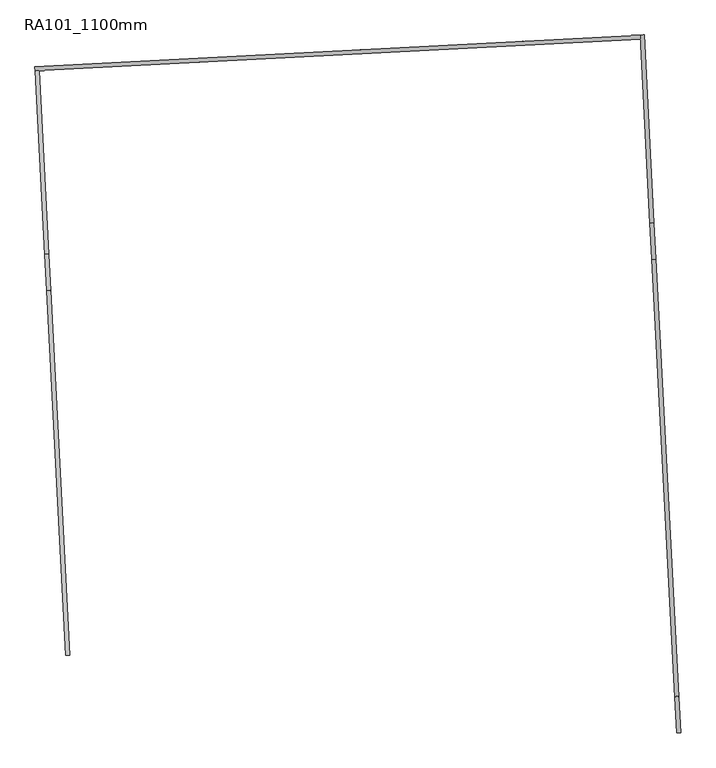
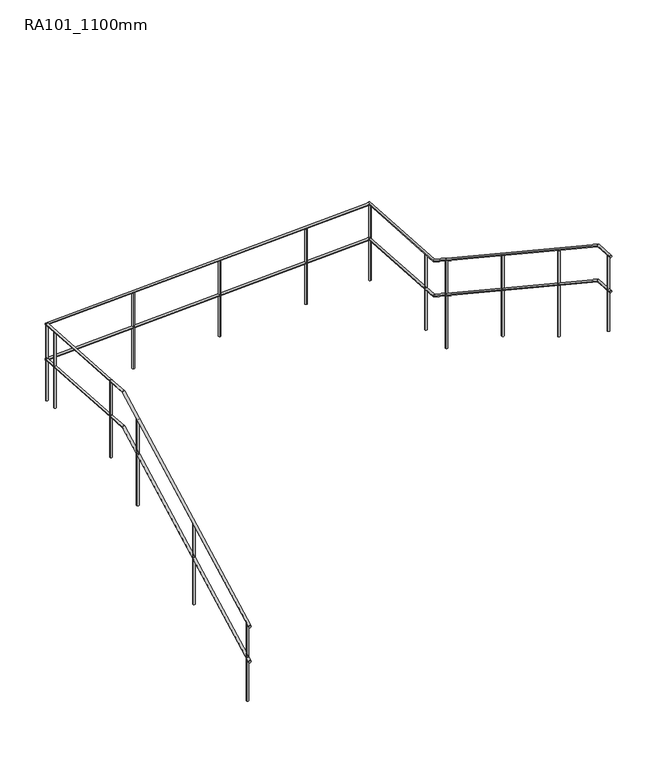
"""IFC4 building model written with IfcOpenShell, lengths in millimetres: railing geometry, RA101_1100mm."""

import ifcopenshell
import ifcopenshell.guid

model = None  # the IFC model being written
_history = None  # IfcOwnerHistory: only IFC2X3 demands one
_inside = {}  # id of a spatial element -> (the spatial element, [elements in it])
_under = {}  # id of a project, library or spatial element -> (it, [spatial elements below it])
_declared = {}  # id of a project -> (the project, [libraries it declares])
_typed = {}  # id of a type object -> (the type object, [elements of that type])
_made_of = {}  # id of a material, layer set ... -> (it, [elements and type objects made of it])


def new_model(schema):
    """Start an empty IFC model of exactly this schema.

    Asked for "IFC4X3", IfcOpenShell would pick the latest addendum, in which some entities
    have other attributes; the version numbers below select the first issue.
    IFC2X3 requires an IfcOwnerHistory on every rooted entity: one is made here for all.
    """
    global model, _history
    if schema == "IFC4X3":
        model = ifcopenshell.file(schema_version=(4, 3, 0, 0))
    else:
        model = ifcopenshell.file(schema=schema)
    _inside.clear()
    _under.clear()
    _declared.clear()
    _typed.clear()
    _made_of.clear()
    _history = None
    if model.schema == "IFC2X3":
        org = make("IfcOrganization", Name="unknown")
        user = make(
            "IfcPersonAndOrganization",
            ThePerson=make("IfcPerson", FamilyName="unknown"),
            TheOrganization=org,
        )
        app = make(
            "IfcApplication",
            ApplicationDeveloper=org,
            Version="unknown",
            ApplicationFullName="unknown",
            ApplicationIdentifier="unknown",
        )
        _history = make(
            "IfcOwnerHistory",
            OwningUser=user,
            OwningApplication=app,
            ChangeAction="ADDED",
            CreationDate=0,
        )
    return model


def make(cls, **values):
    """One entity of the class cls with the attributes given. An attribute that is None is left unset."""
    return model.create_entity(
        cls, **{name: value for name, value in values.items() if value is not None}
    )


def rooted(cls, **values):
    """An entity with a GlobalId (a new one), such as an element, a storey or a relation."""
    return make(cls, GlobalId=ifcopenshell.guid.new(), OwnerHistory=_history, **values)


def si_unit(unit_type, name, prefix=None):
    """IfcSIUnit, for example si_unit("LENGTHUNIT", "METRE", prefix="MILLI")."""
    return make("IfcSIUnit", UnitType=unit_type, Prefix=prefix, Name=name)


def assignment(units):
    """IfcUnitAssignment: the units of a project."""
    return None if units is None else make("IfcUnitAssignment", Units=units)


def point(xyz):
    """IfcCartesianPoint."""
    return None if xyz is None else make("IfcCartesianPoint", Coordinates=xyz)


def direction(xyz):
    """IfcDirection."""
    return None if xyz is None else make("IfcDirection", DirectionRatios=xyz)


def frame(location, z_axis=None, x_axis=None):
    """IfcAxis2Placement3D, a coordinate frame: its origin and axes. An axis left out is left unset."""
    return make(
        "IfcAxis2Placement3D",
        Location=point(location),
        Axis=direction(z_axis),
        RefDirection=direction(x_axis),
    )


def frame_2d(location, x_axis=None):
    """IfcAxis2Placement2D, a coordinate frame in the plane: its origin and x axis."""
    return make(
        "IfcAxis2Placement2D", Location=point(location), RefDirection=direction(x_axis)
    )


def origin():
    """The frame at (0, 0, 0) with its axes left unset."""
    return frame((0.0, 0.0, 0.0))


def place(relative_to, where):
    """IfcLocalPlacement: puts the frame where relative to a parent placement (None: the world)."""
    return make(
        "IfcLocalPlacement", PlacementRelTo=relative_to, RelativePlacement=where
    )


def context(
    kind, dimensions, precision=None, world=None, true_north=None, identifier=None
):
    """IfcGeometricRepresentationContext, for example the 3D "Model" context."""
    return make(
        "IfcGeometricRepresentationContext",
        ContextIdentifier=identifier,
        ContextType=kind,
        CoordinateSpaceDimension=dimensions,
        Precision=precision,
        WorldCoordinateSystem=world,
        TrueNorth=true_north,
    )


def project(units=None, contexts=None):
    """IfcProject with its units and contexts."""
    return rooted(
        "IfcProject",
        Name="project",
        RepresentationContexts=contexts,
        UnitsInContext=assignment(units),
    )


def spatial(cls, under=None, at=None, **own):
    """A site, building, storey or space (cls), placed at a placement, below another one or the project."""
    s = rooted(cls, ObjectPlacement=at, **own)
    if under is not None:
        _under.setdefault(under.id(), (under, []))[1].append(s)
    return s


def circle_curve(where, radius):
    """IfcCircle in the frame where."""
    return make("IfcCircle", Position=where, Radius=radius)


def ellipse_curve(where, semi_axis1, semi_axis2):
    """IfcEllipse in the frame where."""
    return make(
        "IfcEllipse", Position=where, SemiAxis1=semi_axis1, SemiAxis2=semi_axis2
    )


def trimmed(basis, trim1, trim2, sense, master):
    """IfcTrimmedCurve: the piece of a basis curve between two trims."""
    return make(
        "IfcTrimmedCurve",
        BasisCurve=basis,
        Trim1=trim1,
        Trim2=trim2,
        SenseAgreement=sense,
        MasterRepresentation=master,
    )


def segment(curve, same_sense, transition):
    """IfcCompositeCurveSegment."""
    return make(
        "IfcCompositeCurveSegment",
        Transition=transition,
        SameSense=same_sense,
        ParentCurve=curve,
    )


def composite_curve(segments, self_intersect=None):
    """IfcCompositeCurve: segments joined end to end."""
    return make("IfcCompositeCurve", Segments=segments, SelfIntersect=self_intersect)


def outline(outer, holes=None, kind="AREA"):
    """IfcArbitraryClosedProfileDef: a profile drawn as a closed curve; with holes, ...WithVoids."""
    if holes is None:
        return make("IfcArbitraryClosedProfileDef", ProfileType=kind, OuterCurve=outer)
    return make(
        "IfcArbitraryProfileDefWithVoids",
        ProfileType=kind,
        OuterCurve=outer,
        InnerCurves=holes,
    )


def extrude(swept, where, along, depth):
    """IfcExtrudedAreaSolid: the profile swept, set in the frame where, extruded along a direction by depth."""
    return make(
        "IfcExtrudedAreaSolid",
        SweptArea=swept,
        Position=where,
        ExtrudedDirection=direction(along),
        Depth=depth,
    )


def shape(context_of_items, identifier, shape_type, items):
    """IfcShapeRepresentation: the items that make up one representation, for example the "Body"."""
    return make(
        "IfcShapeRepresentation",
        ContextOfItems=context_of_items,
        RepresentationIdentifier=identifier,
        RepresentationType=shape_type,
        Items=items,
    )


def source(mapping_origin, context_of_items, identifier, shape_type, items):
    """IfcRepresentationMap: a shape defined once, which mapped items show again and again."""
    return make(
        "IfcRepresentationMap",
        MappingOrigin=mapping_origin,
        MappedRepresentation=shape(context_of_items, identifier, shape_type, items),
    )


def transform(
    local_origin,
    x_axis=None,
    y_axis=None,
    z_axis=None,
    scale=None,
    scale2=None,
    scale3=None,
    uniform=True,
):
    """IfcCartesianTransformationOperator3D, or its non-uniform kind. x_axis, y_axis, z_axis: its Axis1, 2, 3."""
    if uniform:
        return make(
            "IfcCartesianTransformationOperator3D",
            Axis1=direction(x_axis),
            Axis2=direction(y_axis),
            LocalOrigin=point(local_origin),
            Scale=scale,
            Axis3=direction(z_axis),
        )
    return make(
        "IfcCartesianTransformationOperator3DnonUniform",
        Axis1=direction(x_axis),
        Axis2=direction(y_axis),
        LocalOrigin=point(local_origin),
        Scale=scale,
        Axis3=direction(z_axis),
        Scale2=scale2,
        Scale3=scale3,
    )


def mapped(mapping_source, mapping_target):
    """IfcMappedItem: shows the shape of a source again, moved by a transform."""
    return make(
        "IfcMappedItem", MappingSource=mapping_source, MappingTarget=mapping_target
    )


def made_of(thing, what):
    """Note that an element or type object is made of a material, layer set ...; save() writes the relation."""
    if what is not None:
        _made_of.setdefault(what.id(), (what, []))[1].append(thing)
    return thing


def element(
    cls,
    number,
    at=None,
    inside=None,
    cuts=None,
    type_object=None,
    material=None,
    context=None,
    identifier="Body",
    shape_type=None,
    held_by="IfcProductDefinitionShape",
    body=None,
    shapes=None,
    **own,
):
    """One element of the class cls, such as IfcWall. Its Tag is "e" and its number.

    at: its placement. inside: the storey or other place that contains it. cuts: it is an
    opening in that element (IfcRelVoidsElement). A single representation is given by context,
    identifier, shape_type and body (its items); several are given by shapes. held_by: the class
    of the entity that holds the representations. save() writes the other relations.
    """
    e = rooted(cls, Tag="e%d" % number, ObjectPlacement=at, **own)
    if body is not None:
        shapes = [shape(context, identifier, shape_type, body)]
    if shapes is not None:
        e.Representation = make(held_by, Representations=shapes)
    if inside is not None:
        _inside.setdefault(inside.id(), (inside, []))[1].append(e)
    if cuts is not None:
        rooted(
            "IfcRelVoidsElement", RelatingBuildingElement=cuts, RelatedOpeningElement=e
        )
    if type_object is not None:
        _typed.setdefault(type_object.id(), (type_object, []))[1].append(e)
    return made_of(e, material)


def aggregate(whole, parts):
    """IfcRelAggregates: a whole, such as a stair, and the parts it consists of."""
    return rooted("IfcRelAggregates", RelatingObject=whole, RelatedObjects=parts)


def save(model, path):
    """Write the relations noted so far, then the file.

    IfcRelAggregates (storeys below a building ...), IfcRelContainedInSpatialStructure (elements
    in a storey), IfcRelDefinesByType, IfcRelAssociatesMaterial and IfcRelDeclares: one each for
    every whole, place, type object, material and project.
    """
    for whole, parts in _under.values():
        aggregate(whole, parts)
    for where, things in _inside.values():
        rooted(
            "IfcRelContainedInSpatialStructure",
            RelatedElements=things,
            RelatingStructure=where,
        )
    for kind, things in _typed.values():
        rooted("IfcRelDefinesByType", RelatedObjects=things, RelatingType=kind)
    for what, things in _made_of.values():
        rooted("IfcRelAssociatesMaterial", RelatedObjects=things, RelatingMaterial=what)
    for by, libraries in _declared.values():
        rooted("IfcRelDeclares", RelatingContext=by, RelatedDefinitions=libraries)
    model.write(path)


def plane_surface(at):
    """IfcPlane: the flat surface through the origin of the frame at, square to its z axis."""
    return make("IfcPlane", Position=at)


def cylinder_surface(at, radius):
    """IfcCylindricalSurface: all points at the distance radius from the z axis of the frame at."""
    return make("IfcCylindricalSurface", Position=at, Radius=radius)


def advanced_brep(points, edges, surfaces, faces):
    """IfcAdvancedBrep: a solid bounded by faces that lie on surfaces and meet in shared edges.

    An edge is (start, end): straight between two places in points (the first is 0);
    or (start, end, curve); or (start, end, curve, False) where it runs against its curve.
    A face is (place in surfaces, loops), or (place, loops, False) where it looks against
    its surface's normal. A loop lists edges by number (the first is 1), with a minus sign
    where the edge is run from its end to its start. The first loop is the outer one.
    """
    corners = [point(p) for p in points]
    vertices = [make("IfcVertexPoint", VertexGeometry=c) for c in corners]
    made = []
    for start, end, *more in edges:
        made.append(
            make(
                "IfcEdgeCurve",
                EdgeStart=vertices[start],
                EdgeEnd=vertices[end],
                EdgeGeometry=more[0] if more else make("IfcPolyline", Points=[corners[start], corners[end]]),
                SameSense=more[1] if len(more) > 1 else True,
            )
        )
    hull = []
    for where, loops, *sense in faces:
        bounds = []
        for j, loop in enumerate(loops):
            ring = [make("IfcOrientedEdge", EdgeElement=made[abs(k) - 1], Orientation=k > 0) for k in loop]
            bounds.append(
                make(
                    "IfcFaceOuterBound" if j == 0 else "IfcFaceBound",
                    Bound=make("IfcEdgeLoop", EdgeList=ring),
                    Orientation=True,
                )
            )
        hull.append(make("IfcAdvancedFace", Bounds=bounds, FaceSurface=surfaces[where], SameSense=sense[0] if sense else True))
    return make("IfcAdvancedBrep", Outer=make("IfcClosedShell", CfsFaces=hull))


def ra101_1100mm_925ff370(model_context):
    return source(origin(), model_context, "Body", "SolidModel", [
        advanced_brep(
        [(21553.8210897, 12464.3641407, 457.1248327), (21523.8622036, 12462.794062, 457.1248327), (21412.281847, 15165.0937775, 2210.0), (21382.3229609, 15163.5236988, 2210.0), (21398.3832997, 15430.2938589, 2210.0), (21368.4244136, 15428.7237802, 2210.0)],
        [
            (0, 1, ellipse_curve(frame((21538.8416467, 12463.5791013, 457.1248327), z_axis=(0.052335956242941364, -0.998629534754574, 0.0), x_axis=(0.0, 0.0, -1.0)), 17.8751673, 15.0)),
            (1, 0, ellipse_curve(frame((21538.8416467, 12463.5791013, 457.1248327), z_axis=(0.052335956242941364, -0.998629534754574, 0.0), x_axis=(0.0, 0.0, -1.0)), 17.8751673, 15.0)),
            (0, 2),
            (2, 3, ellipse_curve(frame((21397.302404, 15164.3087382, 2210.0), z_axis=(0.05018733030882, -0.957631309614881, -0.28359038545367027), x_axis=(-0.014841974004008681, 0.2832017346864693, -0.9589455111101147)), 15.6421818, 15.0)),
            (3, 1),
            (3, 2, ellipse_curve(frame((21397.302404, 15164.3087382, 2210.0), z_axis=(0.05018733030882, -0.957631309614881, -0.28359038545367027), x_axis=(-0.014841974004008681, 0.2832017346864693, -0.9589455111101147)), 15.6421818, 15.0)),
            (4, 5, circle_curve(frame((21383.4038566, 15429.5088195, 2210.0), z_axis=(-0.05233595624293373, 0.9986295347545745, 0.0), x_axis=(-0.9986295347545745, -0.05233595624293373, 0.0)), 15.0)),
            (5, 4, circle_curve(frame((21383.4038566, 15429.5088195, 2210.0), z_axis=(-0.05233595624293373, 0.9986295347545745, 0.0), x_axis=(-0.9986295347545745, -0.05233595624293373, 0.0)), 15.0)),
            (2, 4),
            (5, 3),
        ],
        [
            plane_surface(frame((21538.8416467, 12463.5791013, 475.0), z_axis=(0.052335956242941364, -0.998629534754574, 0.0), x_axis=(0.998629534754574, 0.052335956242941364, 0.0))),
            cylinder_surface(frame((21538.4146673, 12471.7263523, 462.4127052), z_axis=(0.04391787398555335, -0.8380029565528062, -0.5438954542495688), x_axis=(-0.998629534754574, -0.05233595624294136, 0.0)), 15.0),
            plane_surface(frame((21383.4038566, 15429.5088195, 2225.0), z_axis=(-0.05233595624293375, 0.9986295347545745, 0.0), x_axis=(0.9986295347545745, 0.05233595624293375, 0.0))),
            cylinder_surface(frame((21397.5345648, 15159.8788452, 2210.0), z_axis=(0.05233595624293373, -0.9986295347545745, 0.0), x_axis=(-0.9986295347545745, -0.05233595624293373, 0.0)), 15.0),
        ],
        [
            (0, [[1, 2]]),
            (1, [[-1, 3, 4, 5]]),
            (1, [[-2, -5, 6, -3]]),
            (2, [[7, 8]]),
            (3, [[-4, 9, -8, 10]]),
            (3, [[-6, -10, -7, -9]]),
        ],
    ),
        advanced_brep(
        [(21398.3832997, 15430.2938589, 2210.0), (21368.4244136, 15428.7237802, 2210.0), (21327.2273335, 16788.0305743, 2210.0), (21297.2684475, 16786.4604957, 2210.0)],
        [
            (0, 1, circle_curve(frame((21383.4038566, 15429.5088195, 2210.0), z_axis=(0.05233595624294149, -0.998629534754574, 0.0), x_axis=(-0.998629534754574, -0.05233595624294149, 0.0)), 15.0)),
            (1, 0, circle_curve(frame((21383.4038566, 15429.5088195, 2210.0), z_axis=(0.05233595624294149, -0.998629534754574, 0.0), x_axis=(-0.998629534754574, -0.05233595624294149, 0.0)), 15.0)),
            (2, 3, circle_curve(frame((21312.2478905, 16787.245535, 2210.0), z_axis=(-0.05233595624294149, 0.998629534754574, 0.0), x_axis=(-0.998629534754574, -0.05233595624294149, 0.0)), 15.0)),
            (3, 2, circle_curve(frame((21312.2478905, 16787.245535, 2210.0), z_axis=(-0.05233595624294149, 0.998629534754574, 0.0), x_axis=(-0.998629534754574, -0.05233595624294149, 0.0)), 15.0)),
            (0, 2),
            (3, 1),
        ],
        [
            plane_surface(frame((21383.4038566, 15429.5088195, 2225.0), z_axis=(0.05233595624294149, -0.998629534754574, 0.0), x_axis=(0.998629534754574, 0.05233595624294149, 0.0))),
            plane_surface(frame((21312.2478905, 16787.245535, 2225.0), z_axis=(-0.05233595624294221, 0.998629534754574, 0.0), x_axis=(0.998629534754574, 0.05233595624294221, 0.0))),
            cylinder_surface(frame((21383.4038566, 15429.5088195, 2210.0), z_axis=(0.05233595624294149, -0.998629534754574, 0.0), x_axis=(-0.998629534754574, -0.05233595624294149, 0.0)), 15.0),
        ],
        [
            (0, [[1, 2]]),
            (1, [[3, 4]]),
            (2, [[-1, 5, -4, 6]]),
            (2, [[-2, -6, -3, -5]]),
        ],
    ),
        advanced_brep(
        [(21297.2684475, 16786.4604957, 2210.0), (21295.6983688, 16816.4193817, 2210.0), (25777.8195811, 17021.2762305, 2210.0), (25776.2495024, 17051.2351166, 2210.0)],
        [
            (0, 1, circle_curve(frame((21296.4834082, 16801.4399387, 2210.0), z_axis=(-0.998629534754574, -0.05233595624294222, 0.0), x_axis=(-0.05233595624294222, 0.998629534754574, 0.0)), 15.0)),
            (1, 0, circle_curve(frame((21296.4834082, 16801.4399387, 2210.0), z_axis=(-0.998629534754574, -0.05233595624294222, 0.0), x_axis=(-0.05233595624294222, 0.998629534754574, 0.0)), 15.0)),
            (2, 3, circle_curve(frame((25777.0345417, 17036.2556736, 2210.0), z_axis=(0.998629534754574, 0.05233595624294222, 0.0), x_axis=(-0.05233595624294222, 0.998629534754574, 0.0)), 15.0)),
            (3, 2, circle_curve(frame((25777.0345417, 17036.2556736, 2210.0), z_axis=(0.998629534754574, 0.05233595624294222, 0.0), x_axis=(-0.05233595624294222, 0.998629534754574, 0.0)), 15.0)),
            (0, 2),
            (3, 1),
        ],
        [
            plane_surface(frame((21296.4834082, 16801.4399387, 2225.0), z_axis=(-0.998629534754574, -0.05233595624294149, 0.0), x_axis=(0.05233595624294149, -0.998629534754574, 0.0))),
            plane_surface(frame((25777.0345417, 17036.2556736, 2225.0), z_axis=(0.9986295347545739, 0.05233595624294333, 0.0), x_axis=(0.05233595624294333, -0.9986295347545739, 0.0))),
            cylinder_surface(frame((21296.4834082, 16801.4399387, 2210.0), z_axis=(-0.998629534754574, -0.05233595624294222, 0.0), x_axis=(-0.05233595624294222, 0.998629534754574, 0.0)), 15.0),
        ],
        [
            (0, [[1, 2]]),
            (1, [[3, 4]]),
            (2, [[-1, 5, -4, 6]]),
            (2, [[-2, -6, -3, -5]]),
        ],
    ),
        advanced_brep(
        [(25776.2495024, 17051.2351166, 2210.0), (25806.2083884, 17052.8051953, 2210.0), (25849.207708, 15659.1096221, 2210.0), (25879.1665941, 15660.6797008, 2210.0), (25863.1062554, 15393.9095407, 2382.1248327), (25893.0651414, 15395.4796194, 2382.1248327)],
        [
            (0, 1, circle_curve(frame((25791.2289454, 17052.0201559, 2210.0), z_axis=(-0.05233595624294333, 0.9986295347545739, 0.0), x_axis=(0.9986295347545739, 0.05233595624294333, 0.0)), 15.0)),
            (1, 0, circle_curve(frame((25791.2289454, 17052.0201559, 2210.0), z_axis=(-0.05233595624294333, 0.9986295347545739, 0.0), x_axis=(0.9986295347545739, 0.05233595624294333, 0.0)), 15.0)),
            (0, 2),
            (2, 3, ellipse_curve(frame((25864.1871511, 15659.8946614, 2210.0), z_axis=(-0.05018733030882886, 0.9576313096148807, -0.2835903854536695), x_axis=(-0.014841974004012624, 0.28320173468646914, 0.9589455111101145)), 15.6421818, 15.0)),
            (3, 1),
            (3, 2, ellipse_curve(frame((25864.1871511, 15659.8946614, 2210.0), z_axis=(-0.05018733030882886, 0.9576313096148807, -0.2835903854536695), x_axis=(-0.014841974004012624, 0.28320173468646914, 0.9589455111101145)), 15.6421818, 15.0)),
            (4, 5, ellipse_curve(frame((25878.0856984, 15394.69458, 2382.1248327), z_axis=(0.05233595624295016, -0.9986295347545736, 0.0), x_axis=(0.0, 0.0, -1.0)), 17.8751673, 15.0)),
            (5, 4, ellipse_curve(frame((25878.0856984, 15394.69458, 2382.1248327), z_axis=(0.05233595624295016, -0.9986295347545736, 0.0), x_axis=(0.0, 0.0, -1.0)), 17.8751673, 15.0)),
            (2, 4),
            (5, 3),
        ],
        [
            plane_surface(frame((25791.2289454, 17052.0201559, 2225.0), z_axis=(-0.05233595624294221, 0.998629534754574, 0.0), x_axis=(0.998629534754574, 0.05233595624294221, 0.0))),
            cylinder_surface(frame((25791.2289454, 17052.0201559, 2210.0), z_axis=(-0.05233595624294333, 0.9986295347545739, 0.0), x_axis=(0.9986295347545739, 0.05233595624294333, 0.0)), 15.0),
            plane_surface(frame((25878.0856984, 15394.69458, 2400.0), z_axis=(0.05233595624295016, -0.9986295347545736, 0.0), x_axis=(0.9986295347545736, 0.05233595624295016, 0.0))),
            cylinder_surface(frame((25864.3819695, 15656.1773035, 2212.4127052), z_axis=(-0.043917873985560775, 0.838002956552807, -0.5438954542495672), x_axis=(0.9986295347545737, 0.05233595624294905, 0.0)), 15.0),
        ],
        [
            (0, [[1, 2]]),
            (1, [[-1, 3, 4, 5]]),
            (1, [[-2, -5, 6, -3]]),
            (2, [[7, 8]]),
            (3, [[-4, 9, -8, 10]]),
            (3, [[-6, -10, -7, -9]]),
        ],
    ),
        advanced_brep(
        [(25863.1062554, 15393.9095407, 2382.1248327), (25893.0651414, 15395.4796194, 2382.1248327), (26032.9069145, 12153.9199551, 4485.0), (26062.8658005, 12155.4900338, 4485.0), (26046.8054618, 11888.7198737, 4485.0), (26076.7643478, 11890.2899524, 4485.0)],
        [
            (0, 1, ellipse_curve(frame((25878.0856984, 15394.69458, 2382.1248327), z_axis=(-0.052335956242941906, 0.998629534754574, 0.0), x_axis=(0.0, 0.0, -1.0)), 17.8751673, 15.0)),
            (1, 0, ellipse_curve(frame((25878.0856984, 15394.69458, 2382.1248327), z_axis=(-0.052335956242941906, 0.998629534754574, 0.0), x_axis=(0.0, 0.0, -1.0)), 17.8751673, 15.0)),
            (0, 2),
            (2, 3, ellipse_curve(frame((26047.8863575, 12154.7049944, 4485.0), z_axis=(-0.05018733030882246, 0.957631309614881, -0.28359038545366994), x_axis=(0.01484197400401534, -0.2832017346864691, -0.9589455111101146)), 15.6421818, 15.0)),
            (3, 1),
            (3, 2, ellipse_curve(frame((26047.8863575, 12154.7049944, 4485.0), z_axis=(-0.05018733030882246, 0.957631309614881, -0.28359038545366994), x_axis=(0.01484197400401534, -0.2832017346864691, -0.9589455111101146)), 15.6421818, 15.0)),
            (4, 5, circle_curve(frame((26061.7849048, 11889.5049131, 4485.0), z_axis=(0.05233595624293795, -0.9986295347545743, 0.0), x_axis=(0.9986295347545743, 0.05233595624293795, 0.0)), 15.0)),
            (5, 4, circle_curve(frame((26061.7849048, 11889.5049131, 4485.0), z_axis=(0.05233595624293795, -0.9986295347545743, 0.0), x_axis=(0.9986295347545743, 0.05233595624293795, 0.0)), 15.0)),
            (2, 4),
            (5, 3),
        ],
        [
            plane_surface(frame((25878.0856984, 15394.69458, 2400.0), z_axis=(-0.052335956242941906, 0.998629534754574, 0.0), x_axis=(0.998629534754574, 0.052335956242941906, 0.0))),
            cylinder_surface(frame((25878.5126777, 15386.5473291, 2387.4127052), z_axis=(-0.04391787398555386, 0.8380029565528069, -0.5438954542495675), x_axis=(0.998629534754574, 0.05233595624294191, 0.0)), 15.0),
            plane_surface(frame((26061.7849048, 11889.5049131, 4500.0), z_axis=(0.05233595624293795, -0.9986295347545743, 0.0), x_axis=(0.9986295347545743, 0.05233595624293795, 0.0))),
            cylinder_surface(frame((26047.6541966, 12159.1348874, 4485.0), z_axis=(-0.05233595624293795, 0.9986295347545743, 0.0), x_axis=(0.9986295347545743, 0.05233595624293795, 0.0)), 15.0),
        ],
        [
            (0, [[1, 2]]),
            (1, [[-1, 3, 4, 5]]),
            (1, [[-2, -5, 6, -3]]),
            (2, [[7, 8]]),
            (3, [[-4, 9, -8, 10]]),
            (3, [[-6, -10, -7, -9]]),
        ],
    ),
        advanced_brep(
        [(21553.8210897, 12464.3641407, 957.1248327), (21523.8622036, 12462.794062, 957.1248327), (21412.281847, 15165.0937775, 2710.0), (21382.3229609, 15163.5236988, 2710.0), (21398.3832997, 15430.2938589, 2710.0), (21368.4244136, 15428.7237802, 2710.0)],
        [
            (0, 1, ellipse_curve(frame((21538.8416467, 12463.5791013, 957.1248327), z_axis=(0.052335956242941364, -0.998629534754574, 0.0), x_axis=(0.0, 0.0, -1.0)), 17.8751673, 15.0)),
            (1, 0, ellipse_curve(frame((21538.8416467, 12463.5791013, 957.1248327), z_axis=(0.052335956242941364, -0.998629534754574, 0.0), x_axis=(0.0, 0.0, -1.0)), 17.8751673, 15.0)),
            (0, 2),
            (2, 3, ellipse_curve(frame((21397.302404, 15164.3087382, 2710.0), z_axis=(0.05018733030882, -0.957631309614881, -0.28359038545367027), x_axis=(-0.014841974004008681, 0.2832017346864693, -0.9589455111101147)), 15.6421818, 15.0)),
            (3, 1),
            (3, 2, ellipse_curve(frame((21397.302404, 15164.3087382, 2710.0), z_axis=(0.05018733030882, -0.957631309614881, -0.28359038545367027), x_axis=(-0.014841974004008681, 0.2832017346864693, -0.9589455111101147)), 15.6421818, 15.0)),
            (4, 5, circle_curve(frame((21383.4038566, 15429.5088195, 2710.0), z_axis=(-0.05233595624293373, 0.9986295347545745, 0.0), x_axis=(-0.9986295347545745, -0.05233595624293373, 0.0)), 15.0)),
            (5, 4, circle_curve(frame((21383.4038566, 15429.5088195, 2710.0), z_axis=(-0.05233595624293373, 0.9986295347545745, 0.0), x_axis=(-0.9986295347545745, -0.05233595624293373, 0.0)), 15.0)),
            (2, 4),
            (5, 3),
        ],
        [
            plane_surface(frame((21538.8416467, 12463.5791013, 975.0), z_axis=(0.052335956242941364, -0.998629534754574, 0.0), x_axis=(0.998629534754574, 0.052335956242941364, 0.0))),
            cylinder_surface(frame((21538.4146673, 12471.7263523, 962.4127052), z_axis=(0.04391787398555335, -0.8380029565528062, -0.5438954542495688), x_axis=(-0.998629534754574, -0.05233595624294136, 0.0)), 15.0),
            plane_surface(frame((21383.4038566, 15429.5088195, 2725.0), z_axis=(-0.05233595624293375, 0.9986295347545745, 0.0), x_axis=(0.9986295347545745, 0.05233595624293375, 0.0))),
            cylinder_surface(frame((21397.5345648, 15159.8788452, 2710.0), z_axis=(0.05233595624293373, -0.9986295347545745, 0.0), x_axis=(-0.9986295347545745, -0.05233595624293373, 0.0)), 15.0),
        ],
        [
            (0, [[1, 2]]),
            (1, [[-1, 3, 4, 5]]),
            (1, [[-2, -5, 6, -3]]),
            (2, [[7, 8]]),
            (3, [[-4, 9, -8, 10]]),
            (3, [[-6, -10, -7, -9]]),
        ],
    ),
        advanced_brep(
        [(21398.3832997, 15430.2938589, 2710.0), (21368.4244136, 15428.7237802, 2710.0), (21327.2273335, 16788.0305743, 2710.0), (21297.2684475, 16786.4604957, 2710.0)],
        [
            (0, 1, circle_curve(frame((21383.4038566, 15429.5088195, 2710.0), z_axis=(0.05233595624294149, -0.998629534754574, 0.0), x_axis=(-0.998629534754574, -0.05233595624294149, 0.0)), 15.0)),
            (1, 0, circle_curve(frame((21383.4038566, 15429.5088195, 2710.0), z_axis=(0.05233595624294149, -0.998629534754574, 0.0), x_axis=(-0.998629534754574, -0.05233595624294149, 0.0)), 15.0)),
            (2, 3, circle_curve(frame((21312.2478905, 16787.245535, 2710.0), z_axis=(-0.05233595624294149, 0.998629534754574, 0.0), x_axis=(-0.998629534754574, -0.05233595624294149, 0.0)), 15.0)),
            (3, 2, circle_curve(frame((21312.2478905, 16787.245535, 2710.0), z_axis=(-0.05233595624294149, 0.998629534754574, 0.0), x_axis=(-0.998629534754574, -0.05233595624294149, 0.0)), 15.0)),
            (0, 2),
            (3, 1),
        ],
        [
            plane_surface(frame((21383.4038566, 15429.5088195, 2725.0), z_axis=(0.05233595624294149, -0.998629534754574, 0.0), x_axis=(0.998629534754574, 0.05233595624294149, 0.0))),
            plane_surface(frame((21312.2478905, 16787.245535, 2725.0), z_axis=(-0.05233595624294221, 0.998629534754574, 0.0), x_axis=(0.998629534754574, 0.05233595624294221, 0.0))),
            cylinder_surface(frame((21383.4038566, 15429.5088195, 2710.0), z_axis=(0.05233595624294149, -0.998629534754574, 0.0), x_axis=(-0.998629534754574, -0.05233595624294149, 0.0)), 15.0),
        ],
        [
            (0, [[1, 2]]),
            (1, [[3, 4]]),
            (2, [[-1, 5, -4, 6]]),
            (2, [[-2, -6, -3, -5]]),
        ],
    ),
        advanced_brep(
        [(21297.2684475, 16786.4604957, 2710.0), (21295.6983688, 16816.4193817, 2710.0), (25777.8195811, 17021.2762305, 2710.0), (25776.2495024, 17051.2351166, 2710.0)],
        [
            (0, 1, circle_curve(frame((21296.4834082, 16801.4399387, 2710.0), z_axis=(-0.998629534754574, -0.05233595624294222, 0.0), x_axis=(-0.05233595624294222, 0.998629534754574, 0.0)), 15.0)),
            (1, 0, circle_curve(frame((21296.4834082, 16801.4399387, 2710.0), z_axis=(-0.998629534754574, -0.05233595624294222, 0.0), x_axis=(-0.05233595624294222, 0.998629534754574, 0.0)), 15.0)),
            (2, 3, circle_curve(frame((25777.0345417, 17036.2556736, 2710.0), z_axis=(0.998629534754574, 0.05233595624294222, 0.0), x_axis=(-0.05233595624294222, 0.998629534754574, 0.0)), 15.0)),
            (3, 2, circle_curve(frame((25777.0345417, 17036.2556736, 2710.0), z_axis=(0.998629534754574, 0.05233595624294222, 0.0), x_axis=(-0.05233595624294222, 0.998629534754574, 0.0)), 15.0)),
            (0, 2),
            (3, 1),
        ],
        [
            plane_surface(frame((21296.4834082, 16801.4399387, 2725.0), z_axis=(-0.998629534754574, -0.05233595624294149, 0.0), x_axis=(0.05233595624294149, -0.998629534754574, 0.0))),
            plane_surface(frame((25777.0345417, 17036.2556736, 2725.0), z_axis=(0.9986295347545739, 0.05233595624294333, 0.0), x_axis=(0.05233595624294333, -0.9986295347545739, 0.0))),
            cylinder_surface(frame((21296.4834082, 16801.4399387, 2710.0), z_axis=(-0.998629534754574, -0.05233595624294222, 0.0), x_axis=(-0.05233595624294222, 0.998629534754574, 0.0)), 15.0),
        ],
        [
            (0, [[1, 2]]),
            (1, [[3, 4]]),
            (2, [[-1, 5, -4, 6]]),
            (2, [[-2, -6, -3, -5]]),
        ],
    ),
        advanced_brep(
        [(25776.2495024, 17051.2351166, 2710.0), (25806.2083884, 17052.8051953, 2710.0), (25849.207708, 15659.1096221, 2710.0), (25879.1665941, 15660.6797008, 2710.0), (25863.1062554, 15393.9095407, 2882.1248327), (25893.0651414, 15395.4796194, 2882.1248327)],
        [
            (0, 1, circle_curve(frame((25791.2289454, 17052.0201559, 2710.0), z_axis=(-0.05233595624294333, 0.9986295347545739, 0.0), x_axis=(0.9986295347545739, 0.05233595624294333, 0.0)), 15.0)),
            (1, 0, circle_curve(frame((25791.2289454, 17052.0201559, 2710.0), z_axis=(-0.05233595624294333, 0.9986295347545739, 0.0), x_axis=(0.9986295347545739, 0.05233595624294333, 0.0)), 15.0)),
            (0, 2),
            (2, 3, ellipse_curve(frame((25864.1871511, 15659.8946614, 2710.0), z_axis=(-0.05018733030882886, 0.9576313096148807, -0.2835903854536695), x_axis=(-0.014841974004012624, 0.28320173468646914, 0.9589455111101145)), 15.6421818, 15.0)),
            (3, 1),
            (3, 2, ellipse_curve(frame((25864.1871511, 15659.8946614, 2710.0), z_axis=(-0.05018733030882886, 0.9576313096148807, -0.2835903854536695), x_axis=(-0.014841974004012624, 0.28320173468646914, 0.9589455111101145)), 15.6421818, 15.0)),
            (4, 5, ellipse_curve(frame((25878.0856984, 15394.69458, 2882.1248327), z_axis=(0.05233595624295016, -0.9986295347545736, 0.0), x_axis=(0.0, 0.0, -1.0)), 17.8751673, 15.0)),
            (5, 4, ellipse_curve(frame((25878.0856984, 15394.69458, 2882.1248327), z_axis=(0.05233595624295016, -0.9986295347545736, 0.0), x_axis=(0.0, 0.0, -1.0)), 17.8751673, 15.0)),
            (2, 4),
            (5, 3),
        ],
        [
            plane_surface(frame((25791.2289454, 17052.0201559, 2725.0), z_axis=(-0.05233595624294221, 0.998629534754574, 0.0), x_axis=(0.998629534754574, 0.05233595624294221, 0.0))),
            cylinder_surface(frame((25791.2289454, 17052.0201559, 2710.0), z_axis=(-0.05233595624294333, 0.9986295347545739, 0.0), x_axis=(0.9986295347545739, 0.05233595624294333, 0.0)), 15.0),
            plane_surface(frame((25878.0856984, 15394.69458, 2900.0), z_axis=(0.05233595624295016, -0.9986295347545736, 0.0), x_axis=(0.9986295347545736, 0.05233595624295016, 0.0))),
            cylinder_surface(frame((25864.3819695, 15656.1773035, 2712.4127052), z_axis=(-0.043917873985560775, 0.838002956552807, -0.5438954542495672), x_axis=(0.9986295347545737, 0.05233595624294905, 0.0)), 15.0),
        ],
        [
            (0, [[1, 2]]),
            (1, [[-1, 3, 4, 5]]),
            (1, [[-2, -5, 6, -3]]),
            (2, [[7, 8]]),
            (3, [[-4, 9, -8, 10]]),
            (3, [[-6, -10, -7, -9]]),
        ],
    ),
        advanced_brep(
        [(25863.1062554, 15393.9095407, 2882.1248327), (25893.0651414, 15395.4796194, 2882.1248327), (26032.9069145, 12153.9199551, 4985.0), (26062.8658005, 12155.4900338, 4985.0), (26046.8054618, 11888.7198737, 4985.0), (26076.7643478, 11890.2899524, 4985.0)],
        [
            (0, 1, ellipse_curve(frame((25878.0856984, 15394.69458, 2882.1248327), z_axis=(-0.052335956242941906, 0.998629534754574, 0.0), x_axis=(0.0, 0.0, -1.0)), 17.8751673, 15.0)),
            (1, 0, ellipse_curve(frame((25878.0856984, 15394.69458, 2882.1248327), z_axis=(-0.052335956242941906, 0.998629534754574, 0.0), x_axis=(0.0, 0.0, -1.0)), 17.8751673, 15.0)),
            (0, 2),
            (2, 3, ellipse_curve(frame((26047.8863575, 12154.7049944, 4985.0), z_axis=(-0.05018733030882246, 0.957631309614881, -0.28359038545366994), x_axis=(0.01484197400401534, -0.2832017346864691, -0.9589455111101146)), 15.6421818, 15.0)),
            (3, 1),
            (3, 2, ellipse_curve(frame((26047.8863575, 12154.7049944, 4985.0), z_axis=(-0.05018733030882246, 0.957631309614881, -0.28359038545366994), x_axis=(0.01484197400401534, -0.2832017346864691, -0.9589455111101146)), 15.6421818, 15.0)),
            (4, 5, circle_curve(frame((26061.7849048, 11889.5049131, 4985.0), z_axis=(0.05233595624293795, -0.9986295347545743, 0.0), x_axis=(0.9986295347545743, 0.05233595624293795, 0.0)), 15.0)),
            (5, 4, circle_curve(frame((26061.7849048, 11889.5049131, 4985.0), z_axis=(0.05233595624293795, -0.9986295347545743, 0.0), x_axis=(0.9986295347545743, 0.05233595624293795, 0.0)), 15.0)),
            (2, 4),
            (5, 3),
        ],
        [
            plane_surface(frame((25878.0856984, 15394.69458, 2900.0), z_axis=(-0.052335956242941906, 0.998629534754574, 0.0), x_axis=(0.998629534754574, 0.052335956242941906, 0.0))),
            cylinder_surface(frame((25878.5126777, 15386.5473291, 2887.4127052), z_axis=(-0.04391787398555386, 0.8380029565528069, -0.5438954542495675), x_axis=(0.998629534754574, 0.05233595624294191, 0.0)), 15.0),
            plane_surface(frame((26061.7849048, 11889.5049131, 5000.0), z_axis=(0.05233595624293795, -0.9986295347545743, 0.0), x_axis=(0.9986295347545743, 0.05233595624293795, 0.0))),
            cylinder_surface(frame((26047.6541966, 12159.1348874, 4985.0), z_axis=(-0.05233595624293795, 0.9986295347545743, 0.0), x_axis=(0.9986295347545743, 0.05233595624293795, 0.0)), 15.0),
        ],
        [
            (0, [[1, 2]]),
            (1, [[-1, 3, 4, 5]]),
            (1, [[-2, -5, 6, -3]]),
            (2, [[7, 8]]),
            (3, [[-4, 9, -8, 10]]),
            (3, [[-6, -10, -7, -9]]),
        ],
    ),
        extrude(outline(composite_curve([segment(trimmed(circle_curve(frame_2d((26003.6919934, 12997.9836966)), 15.0), [point((26018.6714364, 12998.768736))], [point((25988.7125504, 12997.1986573))], False, "CARTESIAN"), True, "CONTINUOUS"), segment(trimmed(circle_curve(frame_2d((26003.6919934, 12997.9836966)), 15.0), [point((25988.7125504, 12997.1986573))], [point((26018.6714364, 12998.768736))], False, "CARTESIAN"), True, "CONTINUOUS")], self_intersect=False)), frame((0.0, 0.0, 3200.0), z_axis=(0.0, 0.0, 1.0), x_axis=(1.0, 0.0, 0.0)), (0.0, 0.0, 1.0), 1225.5555556),
        extrude(outline(composite_curve([segment(trimmed(circle_curve(frame_2d((25940.8888459, 14196.3391383)), 15.0), [point((25955.8682889, 14197.1241777))], [point((25925.9094029, 14195.554099))], False, "CARTESIAN"), True, "CONTINUOUS"), segment(trimmed(circle_curve(frame_2d((25940.8888459, 14196.3391383)), 15.0), [point((25925.9094029, 14195.554099))], [point((25955.8682889, 14197.1241777))], False, "CARTESIAN"), True, "CONTINUOUS")], self_intersect=False)), frame((0.0, 0.0, 2500.0), z_axis=(0.0, 0.0, 1.0), x_axis=(1.0, 0.0, 0.0)), (0.0, 0.0, 1.0), 1147.7777778),
        extrude(outline(composite_curve([segment(trimmed(circle_curve(frame_2d((25854.8171323, 15838.6852712)), 15.0), [point((25869.7965753, 15839.4703105))], [point((25839.8376892, 15837.9002318))], False, "CARTESIAN"), True, "CONTINUOUS"), segment(trimmed(circle_curve(frame_2d((25854.8171323, 15838.6852712)), 15.0), [point((25839.8376892, 15837.9002318))], [point((25869.7965753, 15839.4703105))], False, "CARTESIAN"), True, "CONTINUOUS")], self_intersect=False)), frame((0.0, 0.0, 1625.0), z_axis=(0.0, 0.0, 1.0), x_axis=(1.0, 0.0, 0.0)), (0.0, 0.0, 1.0), 1070.0),
        extrude(outline(composite_curve([segment(trimmed(circle_curve(frame_2d((24906.5291763, 16990.6344205)), 15.0), [point((24905.744137, 17005.6138635))], [point((24907.3142156, 16975.6549775))], False, "CARTESIAN"), True, "CONTINUOUS"), segment(trimmed(circle_curve(frame_2d((24906.5291763, 16990.6344205)), 15.0), [point((24907.3142156, 16975.6549775))], [point((24905.744137, 17005.6138635))], False, "CARTESIAN"), True, "CONTINUOUS")], self_intersect=False)), frame((0.0, 0.0, 1625.0), z_axis=(0.0, 0.0, 1.0), x_axis=(1.0, 0.0, 0.0)), (0.0, 0.0, 1.0), 1070.0),
        extrude(outline(composite_curve([segment(trimmed(circle_curve(frame_2d((23708.1737346, 16927.831273)), 15.0), [point((23707.3886952, 16942.810716))], [point((23708.9587739, 16912.85183))], False, "CARTESIAN"), True, "CONTINUOUS"), segment(trimmed(circle_curve(frame_2d((23708.1737346, 16927.831273)), 15.0), [point((23708.9587739, 16912.85183))], [point((23707.3886952, 16942.810716))], False, "CARTESIAN"), True, "CONTINUOUS")], self_intersect=False)), frame((0.0, 0.0, 1625.0), z_axis=(0.0, 0.0, 1.0), x_axis=(1.0, 0.0, 0.0)), (0.0, 0.0, 1.0), 1070.0),
        extrude(outline(composite_curve([segment(trimmed(circle_curve(frame_2d((22509.8182929, 16865.0281255)), 15.0), [point((22509.0332535, 16880.0075685))], [point((22510.6033322, 16850.0486825))], False, "CARTESIAN"), True, "CONTINUOUS"), segment(trimmed(circle_curve(frame_2d((22509.8182929, 16865.0281255)), 15.0), [point((22510.6033322, 16850.0486825))], [point((22509.0332535, 16880.0075685))], False, "CARTESIAN"), True, "CONTINUOUS")], self_intersect=False)), frame((0.0, 0.0, 1625.0), z_axis=(0.0, 0.0, 1.0), x_axis=(1.0, 0.0, 0.0)), (0.0, 0.0, 1.0), 1070.0),
        extrude(outline(composite_curve([segment(trimmed(circle_curve(frame_2d((21320.6007091, 16627.8642613)), 15.0), [point((21305.6212661, 16627.0792219))], [point((21335.5801522, 16628.6493006))], False, "CARTESIAN"), True, "CONTINUOUS"), segment(trimmed(circle_curve(frame_2d((21320.6007091, 16627.8642613)), 15.0), [point((21335.5801522, 16628.6493006))], [point((21305.6212661, 16627.0792219))], False, "CARTESIAN"), True, "CONTINUOUS")], self_intersect=False)), frame((0.0, 0.0, 1625.0), z_axis=(0.0, 0.0, 1.0), x_axis=(1.0, 0.0, 0.0)), (0.0, 0.0, 1.0), 1070.0),
        extrude(outline(composite_curve([segment(trimmed(circle_curve(frame_2d((21413.2353517, 14860.2899847)), 15.0), [point((21398.2559087, 14859.5049454))], [point((21428.2147947, 14861.0750241))], False, "CARTESIAN"), True, "CONTINUOUS"), segment(trimmed(circle_curve(frame_2d((21413.2353517, 14860.2899847)), 15.0), [point((21428.2147947, 14861.0750241))], [point((21398.2559087, 14859.5049454))], False, "CARTESIAN"), True, "CONTINUOUS")], self_intersect=False)), frame((0.0, 0.0, 1275.0), z_axis=(0.0, 0.0, 1.0), x_axis=(1.0, 0.0, 0.0)), (0.0, 0.0, 1.0), 1225.5555556),
        extrude(outline(composite_curve([segment(trimmed(circle_curve(frame_2d((21476.0384992, 13661.934543)), 15.0), [point((21461.0590562, 13661.1495037))], [point((21491.0179422, 13662.7195824))], False, "CARTESIAN"), True, "CONTINUOUS"), segment(trimmed(circle_curve(frame_2d((21476.0384992, 13661.934543)), 15.0), [point((21491.0179422, 13662.7195824))], [point((21461.0590562, 13661.1495037))], False, "CARTESIAN"), True, "CONTINUOUS")], self_intersect=False)), frame((0.0, 0.0, 575.0), z_axis=(0.0, 0.0, 1.0), x_axis=(1.0, 0.0, 0.0)), (0.0, 0.0, 1.0), 1147.7777778),
        extrude(outline(composite_curve([segment(trimmed(circle_curve(frame_2d((25878.0856984, 15394.69458)), 15.0), [point((25893.0651414, 15395.4796194))], [point((25863.1062554, 15393.9095407))], False, "CARTESIAN"), True, "CONTINUOUS"), segment(trimmed(circle_curve(frame_2d((25878.0856984, 15394.69458)), 15.0), [point((25863.1062554, 15393.9095407))], [point((25893.0651414, 15395.4796194))], False, "CARTESIAN"), True, "CONTINUOUS")], self_intersect=False)), frame((0.0, 0.0, 1625.0), z_axis=(0.0, 0.0, 1.0), x_axis=(1.0, 0.0, 0.0)), (0.0, 0.0, 1.0), 1245.0),
        extrude(outline(composite_curve([segment(trimmed(circle_curve(frame_2d((25792.0139848, 17037.0407129)), 15.0), [point((25791.2289454, 17052.0201559))], [point((25792.7990241, 17022.0612699))], False, "CARTESIAN"), True, "CONTINUOUS"), segment(trimmed(circle_curve(frame_2d((25792.0139848, 17037.0407129)), 15.0), [point((25792.7990241, 17022.0612699))], [point((25791.2289454, 17052.0201559))], False, "CARTESIAN"), True, "CONTINUOUS")], self_intersect=False)), frame((0.0, 0.0, 1625.0), z_axis=(0.0, 0.0, 1.0), x_axis=(1.0, 0.0, 0.0)), (0.0, 0.0, 1.0), 1070.0),
        extrude(outline(composite_curve([segment(trimmed(circle_curve(frame_2d((21311.4628512, 16802.224978)), 15.0), [point((21296.4834082, 16801.4399387))], [point((21326.4422942, 16803.0100174))], False, "CARTESIAN"), True, "CONTINUOUS"), segment(trimmed(circle_curve(frame_2d((21311.4628512, 16802.224978)), 15.0), [point((21326.4422942, 16803.0100174))], [point((21296.4834082, 16801.4399387))], False, "CARTESIAN"), True, "CONTINUOUS")], self_intersect=False)), frame((0.0, 0.0, 1625.0), z_axis=(0.0, 0.0, 1.0), x_axis=(1.0, 0.0, 0.0)), (0.0, 0.0, 1.0), 1070.0),
        extrude(outline(composite_curve([segment(trimmed(circle_curve(frame_2d((21383.4038566, 15429.5088195)), 15.0), [point((21368.4244136, 15428.7237802))], [point((21398.3832997, 15430.2938589))], False, "CARTESIAN"), True, "CONTINUOUS"), segment(trimmed(circle_curve(frame_2d((21383.4038566, 15429.5088195)), 15.0), [point((21398.3832997, 15430.2938589))], [point((21368.4244136, 15428.7237802))], False, "CARTESIAN"), True, "CONTINUOUS")], self_intersect=False)), frame((0.0, 0.0, 1625.0), z_axis=(0.0, 0.0, 1.0), x_axis=(1.0, 0.0, 0.0)), (0.0, 0.0, 1.0), 1070.0),
        extrude(outline(composite_curve([segment(trimmed(circle_curve(frame_2d((26059.168107, 11939.4363898)), 15.0), [point((26074.14755, 11940.2214291))], [point((26044.188664, 11938.6513504))], False, "CARTESIAN"), True, "CONTINUOUS"), segment(trimmed(circle_curve(frame_2d((26059.168107, 11939.4363898)), 15.0), [point((26044.188664, 11938.6513504))], [point((26074.14755, 11940.2214291))], False, "CARTESIAN"), True, "CONTINUOUS")], self_intersect=False)), frame((0.0, 0.0, 3900.0), z_axis=(0.0, 0.0, 1.0), x_axis=(1.0, 0.0, 0.0)), (0.0, 0.0, 1.0), 1070.0),
        extrude(outline(composite_curve([segment(trimmed(circle_curve(frame_2d((21536.2248489, 12513.5105781)), 15.0), [point((21521.2454058, 12512.7255387))], [point((21551.2042919, 12514.2956174))], False, "CARTESIAN"), True, "CONTINUOUS"), segment(trimmed(circle_curve(frame_2d((21536.2248489, 12513.5105781)), 15.0), [point((21551.2042919, 12514.2956174))], [point((21521.2454058, 12512.7255387))], False, "CARTESIAN"), True, "CONTINUOUS")], self_intersect=False)), frame((0.0, 0.0, -125.0), z_axis=(0.0, 0.0, 1.0), x_axis=(1.0, 0.0, 0.0)), (0.0, 0.0, 1.0), 1102.4074074),
    ])


if __name__ == "__main__":
    model = new_model("IFC4")
    model_context = context("Model", 3, world=origin())
    ifc_project = project(units=[si_unit("LENGTHUNIT", "METRE", prefix="MILLI")], contexts=[model_context])
    site = spatial("IfcSite", under=ifc_project)
    building = spatial("IfcBuilding", under=site)
    placement = place(None, origin())
    ra101_1100mm_shape = ra101_1100mm_925ff370(model_context)
    element("IfcRailing", 1, ObjectType="RA101_1100mm", at=placement, inside=building, context=model_context, shape_type="MappedRepresentation", body=[
        mapped(ra101_1100mm_shape, transform((0.0, 0.0, 0.0), x_axis=(1.0, 0.0, 0.0), y_axis=(0.0, 1.0, 0.0), z_axis=(0.0, 0.0, 1.0))),
    ])
    save(model, "model.ifc")
